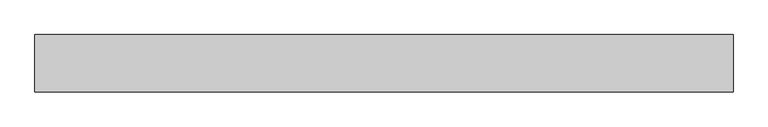
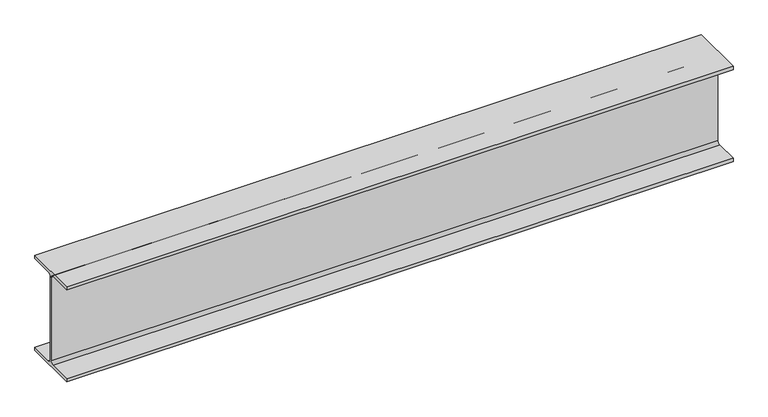
"""IFC4 building model written with IfcOpenShell, lengths in millimetres: beam geometry, Old_Steel Beam_H-KSD3502 : H_SB_ASB_H-194×150x6x9."""

from ifc_helpers import new_model, si_unit, point, frame, frame_2d, origin, place, context, project, spatial, polyline, circle_curve, trimmed, segment, composite_curve, outline, extrude, source, transform, mapped, element, save


def beam_bab581fe(model_context):
    return source(origin(), model_context, "Body", "SweptSolid", [
        extrude(outline(composite_curve([segment(polyline([(-82.5, -141.5), (-11.9, -141.5)]), True, "CONTINUOUS"), segment(trimmed(circle_curve(frame_2d((-11.9, -132.6)), 8.9), [point((-11.9, -141.5))], [point((-3.0, -132.6))], True, "CARTESIAN"), True, "CONTINUOUS"), segment(polyline([(-3.0, -132.6), (-3.0, 132.6)]), True, "CONTINUOUS"), segment(trimmed(circle_curve(frame_2d((-11.9, 132.6)), 8.9), [point((-3.0, 132.6))], [point((-11.9, 141.5))], True, "CARTESIAN"), True, "CONTINUOUS"), segment(polyline([(-11.9, 141.5), (-82.5, 141.5), (-82.5, 151.7), (82.5, 151.7), (82.5, 141.5), (11.9, 141.5)]), True, "CONTINUOUS"), segment(trimmed(circle_curve(frame_2d((11.9, 132.6)), 8.9), [point((11.9, 141.5))], [point((3.0, 132.6))], True, "CARTESIAN"), True, "CONTINUOUS"), segment(polyline([(3.0, 132.6), (3.0, -132.6)]), True, "CONTINUOUS"), segment(trimmed(circle_curve(frame_2d((11.9, -132.6)), 8.9), [point((3.0, -132.6))], [point((11.9, -141.5))], True, "CARTESIAN"), True, "CONTINUOUS"), segment(polyline([(11.9, -141.5), (82.5, -141.5), (82.5, -151.7), (-82.5, -151.7), (-82.5, -141.5)]), True, "CONTINUOUS")], self_intersect=False)), frame((-1117.4837616, 0.0, 0.0), z_axis=(1.0, 0.0, 0.0), x_axis=(0.0, 1.0, 0.0)), (0.0, 0.0, 1.0), 2006.3303739),
    ])


if __name__ == "__main__":
    model = new_model("IFC4")
    model_context = context("Model", 3, world=origin())
    ifc_project = project(units=[si_unit("LENGTHUNIT", "METRE", prefix="MILLI")], contexts=[model_context])
    site = spatial("IfcSite", under=ifc_project)
    building = spatial("IfcBuilding", under=site)
    placement = place(None, origin())
    beam_shape = beam_bab581fe(model_context)
    element("IfcBeam", 1, ObjectType="Old_Steel Beam_H-KSD3502 : H_SB_ASB_H-194×150x6x9", at=placement, inside=building, context=model_context, shape_type="MappedRepresentation", body=[
        mapped(beam_shape, transform((0.0, 0.0, 0.0), x_axis=(1.0, 0.0, 0.0), y_axis=(0.0, 1.0, 0.0), z_axis=(0.0, 0.0, 1.0))),
    ])
    save(model, "model.ifc")

# Revit data of these elements
# Type "Old_Steel Beam_H-KSD3502 : H_SB_ASB_H-194×150x6x9"
#   Width = 15.0 cm
#   Web Thickness = 0.6 cm
#   Web Fillet = 1.3 cm
#   Warping Constant = 43316.0 cm⁶
#   Torsional Moment of Inertia = 8.622 cm⁴
#   Torsional Modulus = 1.0 cm³
#   Section Area = 39.01 cm²
#   Plastic Modulus weak axis = 104.0 cm³
#   Plastic Modulus strong axis = 309.0 cm³
#   Perimeter = 0.95 m²/m
#   Nominal Weight = 30.60 kgf/m
#   Moment of Inertia weak axis = 507.00 cm⁴
#   Moment of Inertia strong axis = 2690.00 cm⁴
#   Height = 19.4 cm
#   Flange Thickness = 0.9 cm
#   Elastic Modulus weak axis = 67.6 cm³
#   Elastic Modulus strong axis = 277.0 cm³
#   Centroid Vertical = 9.7 cm
#   Centroid Horizontal = 7.5 cm
#   Length [instance default] = 1.5240 m
#   Structural Material [instance default] = Steel, 45-345
#   Assembly Code = ""
# Element 1 (IfcBeam, "Old_Steel Beam_H-KSD3502 : H_SB_ASB_H-194×150x6x9")
#   Structural Material = none
# Materials
#   "Steel, 45-345": class "Metal", colour RGB 189 187 185, transparency 0, Description = "Steel 345 MPa", Cost = 0
